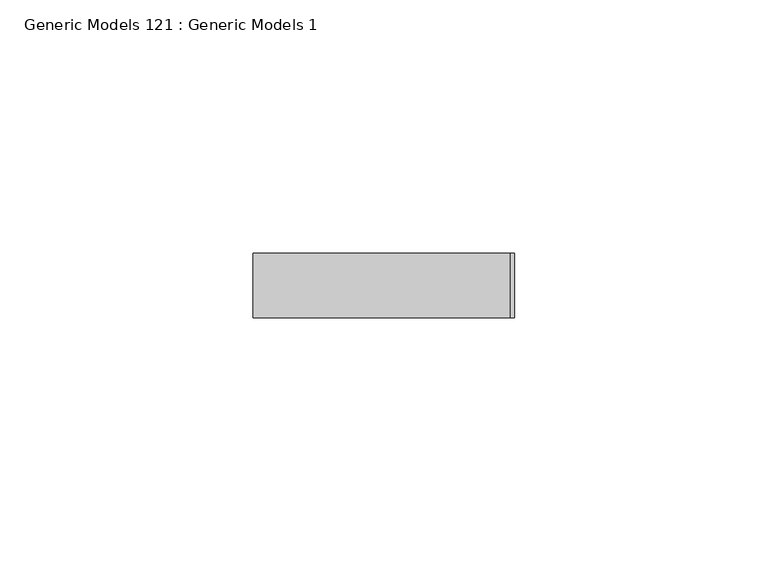
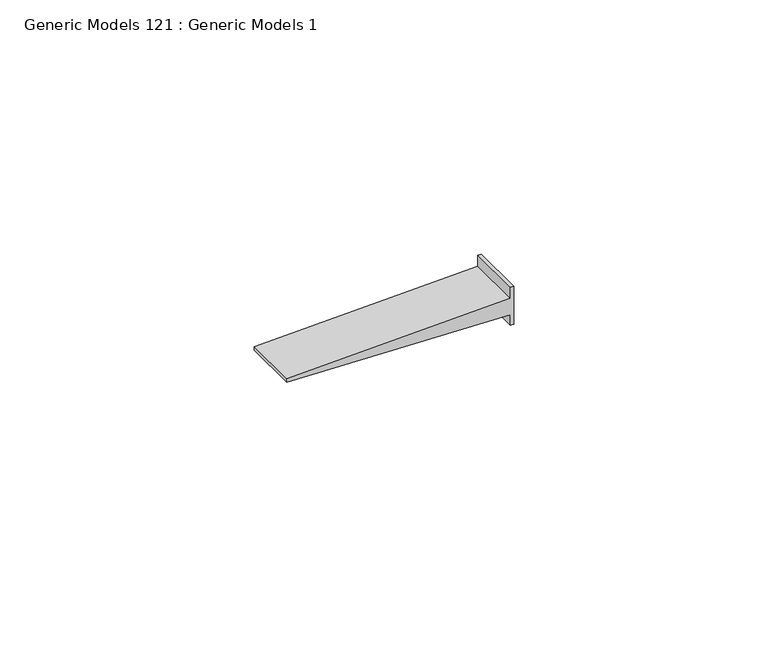
"""IFC4 building model written with IfcOpenShell, lengths in millimetres: proxy geometry, Generic Models 121 : Generic Models 1."""

from ifc_helpers import new_model, si_unit, frame, origin, place, context, project, spatial, polyline, outline, extrude, source, transform, mapped, element, save


def generic_models_121_generic_models_1_ae7d0063(model_context):
    return source(origin(), model_context, "Body", "SweptSolid", [
        extrude(outline(polyline([(2183.633033, 46952.5423031), (2183.633033, 46951.7485531), (2181.0831694, 46951.7485531), (2179.4857803, 46900.9485531), (2178.6870857, 46900.9485531), (2177.0896966, 46951.7485531), (2174.539833, 46951.7485531), (2174.539833, 46952.5423031), (2183.633033, 46952.5423031)])), frame((0.0, 565.15, 0.0), z_axis=(0.0, 1.0, 0.0), x_axis=(0.0, 0.0, 1.0)), (0.0, 0.0, 1.0), 12.7),
    ])


if __name__ == "__main__":
    model = new_model("IFC4")
    model_context = context("Model", 3, world=origin())
    ifc_project = project(units=[si_unit("LENGTHUNIT", "METRE", prefix="MILLI")], contexts=[model_context])
    site = spatial("IfcSite", under=ifc_project)
    building = spatial("IfcBuilding", under=site)
    placement = place(None, origin())
    generic_models_121_generic_models_1_shape = generic_models_121_generic_models_1_ae7d0063(model_context)
    element("IfcBuildingElementProxy", 1, Name="Generic Models 121 : Generic Models 1", ObjectType="Generic Models 121 : Generic Models 1", at=placement, inside=building, context=model_context, shape_type="MappedRepresentation", body=[
        mapped(generic_models_121_generic_models_1_shape, transform((0.0, 0.0, 0.0), x_axis=(1.0, 0.0, 0.0), y_axis=(0.0, 1.0, 0.0), z_axis=(0.0, 0.0, 1.0))),
    ])
    save(model, "model.ifc")

# Revit data of these elements
# Element 1 (IfcBuildingElementProxy, "Generic Models 121 : Generic Models 1")
#   Materials on its faces: "ATTACH GYPSUM BOARD TO STUDS AND NOT TO TOP TRACK"
# Materials
#   "ATTACH GYPSUM BOARD TO STUDS AND NOT TO TOP TRACK": class "Generic", colour RGB 48 48 48, transparency 0, Cost = 0
